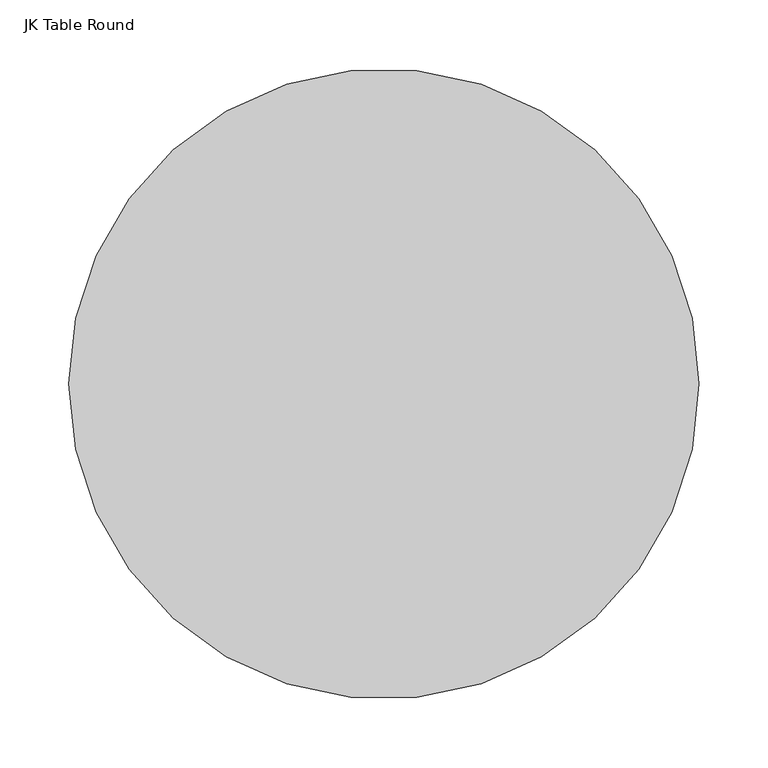
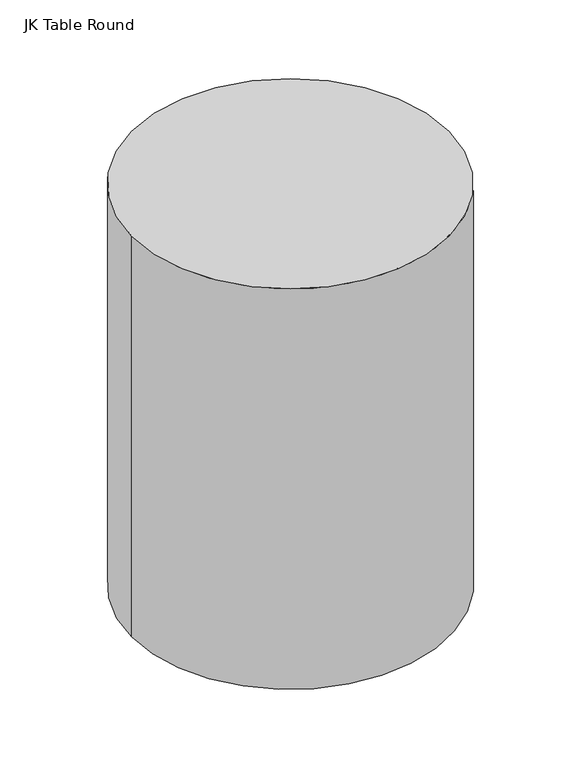
"""IFC4 building model written with IfcOpenShell, lengths in millimetres: furniture geometry, JK Table Round : Counsel End Table."""

from ifc_helpers import new_model, si_unit, point, frame_2d, origin, origin_with_axes, place, context, project, spatial, circle_curve, trimmed, segment, composite_curve, outline, extrude, source, transform, mapped, element, save


def jk_table_round_8e4beac5(model_context):
    return source(origin(), model_context, "Body", "SweptSolid", [
        extrude(outline(composite_curve([segment(trimmed(circle_curve(frame_2d((-61.9426335, 33.5455296)), 228.6), [point((-290.5426335, 33.5455296))], [point((166.6573665, 33.5455296))], False, "CARTESIAN"), True, "CONTINUOUS"), segment(trimmed(circle_curve(frame_2d((-61.9426335, 33.5455296)), 228.6), [point((166.6573665, 33.5455296))], [point((-290.5426335, 33.5455296))], False, "CARTESIAN"), True, "CONTINUOUS")], self_intersect=False)), origin_with_axes(), (0.0, 0.0, 1.0), 609.6),
    ])


if __name__ == "__main__":
    model = new_model("IFC4")
    model_context = context("Model", 3, world=origin())
    ifc_project = project(units=[si_unit("LENGTHUNIT", "METRE", prefix="MILLI")], contexts=[model_context])
    site = spatial("IfcSite", under=ifc_project)
    building = spatial("IfcBuilding", under=site)
    placement = place(None, origin())
    jk_table_round_shape = jk_table_round_8e4beac5(model_context)
    element("IfcFurniture", 1, ObjectType="JK Table Round : Counsel End Table", at=placement, inside=building, context=model_context, shape_type="MappedRepresentation", body=[
        mapped(jk_table_round_shape, transform((0.0, 0.0, 0.0), x_axis=(1.0, 0.0, 0.0), y_axis=(0.0, 1.0, 0.0), z_axis=(0.0, 0.0, 1.0))),
    ])
    save(model, "model.ifc")

# Revit data of these elements
# Type "JK Table Round : Counsel End Table"
#   Width = 1' - 6"
#   Height = 2' - 0"
#   Status [instance default] = none
#   Default Elevation = 0
